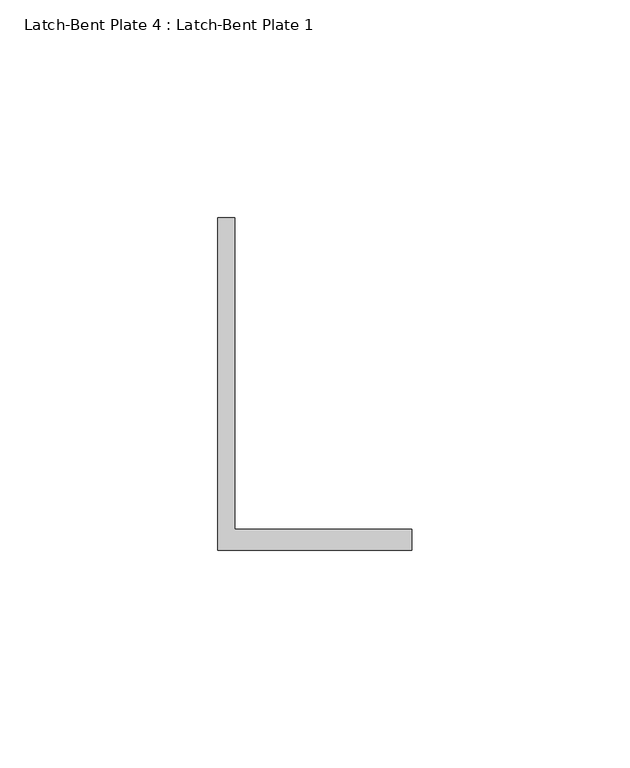
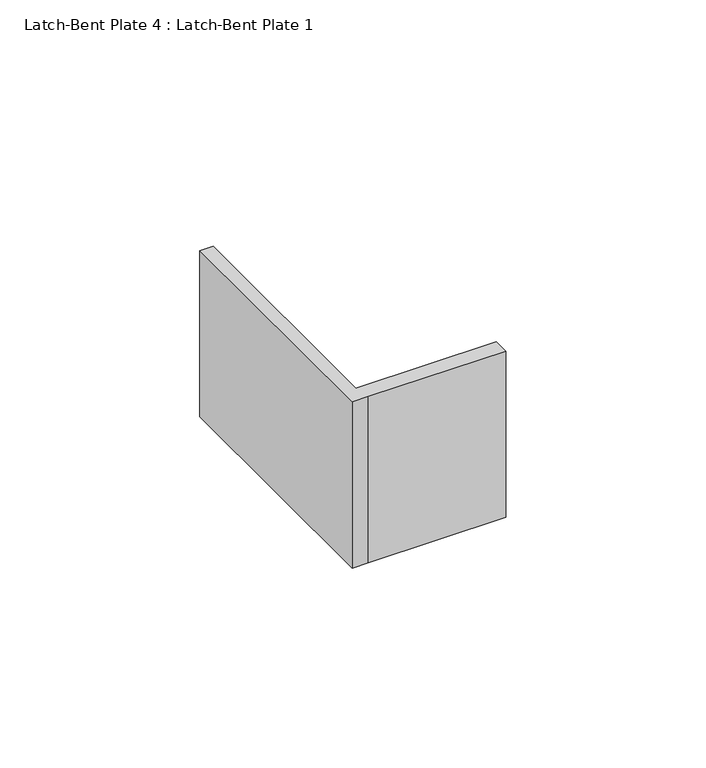
"""IFC4 building model written with IfcOpenShell, lengths in millimetres: proxy geometry, Latch-Bent Plate 4 : Latch-Bent Plate 1."""

from ifc_helpers import new_model, si_unit, frame, origin, place, context, project, spatial, polyline, outline, extrude, source, transform, mapped, element, save


def latch_bent_plate_4_latch_bent_plate_1_9e542a81(model_context):
    return source(origin(), model_context, "Body", "SweptSolid", [
        extrude(outline(polyline([(587327.0060739, -535201.5663841), (587322.2435739, -535201.5663841), (587322.2435739, -535125.3663841), (587326.1141748, -535125.3663841), (587326.1141748, -535196.8038841), (587366.6808739, -535196.8038841), (587366.6808739, -535201.5663841), (587327.0060739, -535201.5663841)])), frame((0.0, 0.0, 1041.4), z_axis=(0.0, 0.0, 1.0), x_axis=(1.0, 0.0, 0.0)), (0.0, 0.0, 1.0), 50.8),
    ])


if __name__ == "__main__":
    model = new_model("IFC4")
    model_context = context("Model", 3, world=origin())
    ifc_project = project(units=[si_unit("LENGTHUNIT", "METRE", prefix="MILLI")], contexts=[model_context])
    site = spatial("IfcSite", under=ifc_project)
    building = spatial("IfcBuilding", under=site)
    placement = place(None, origin())
    latch_bent_plate_4_latch_bent_plate_1_shape = latch_bent_plate_4_latch_bent_plate_1_9e542a81(model_context)
    element("IfcBuildingElementProxy", 1, Name="Latch-Bent Plate 4 : Latch-Bent Plate 1", ObjectType="Latch-Bent Plate 4 : Latch-Bent Plate 1", at=placement, inside=building, context=model_context, shape_type="MappedRepresentation", body=[
        mapped(latch_bent_plate_4_latch_bent_plate_1_shape, transform((0.0, 0.0, 0.0), x_axis=(1.0, 0.0, 0.0), y_axis=(0.0, 1.0, 0.0), z_axis=(0.0, 0.0, 1.0))),
    ])
    save(model, "model.ifc")

# Revit data of these elements
# Element 1 (IfcBuildingElementProxy, "Latch-Bent Plate 4 : Latch-Bent Plate 1")
#   Materials on its faces: "GALV. GATE LATCH"
# Materials
#   "GALV. GATE LATCH": class "Metal", colour RGB 189 187 185, transparency 0, Description = "Carbon steel", Cost = 0
